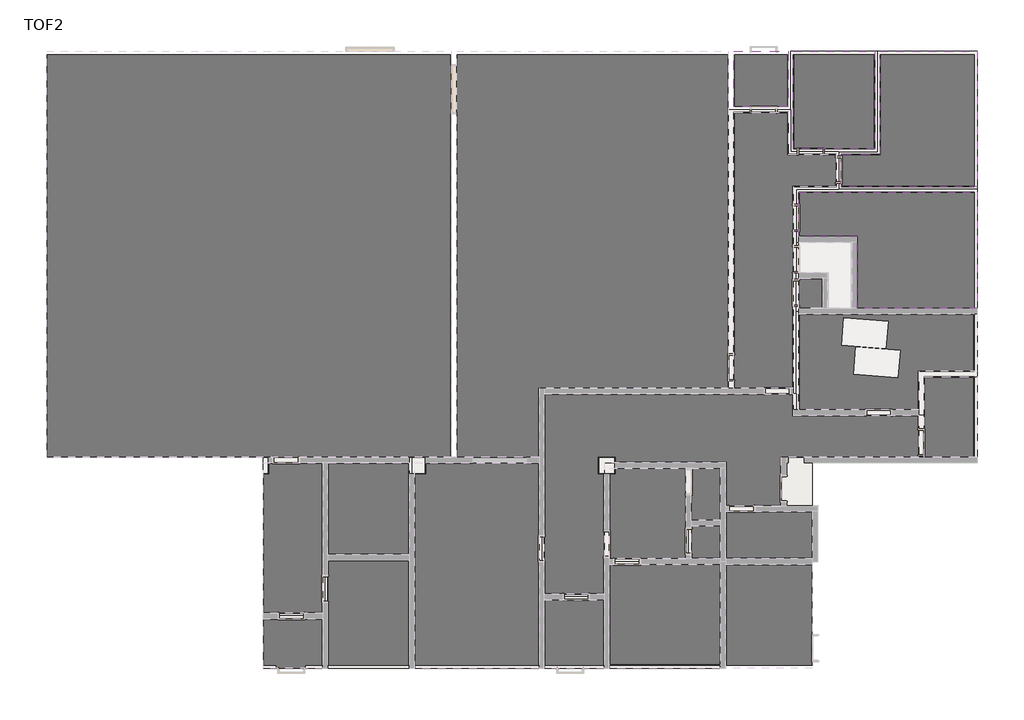
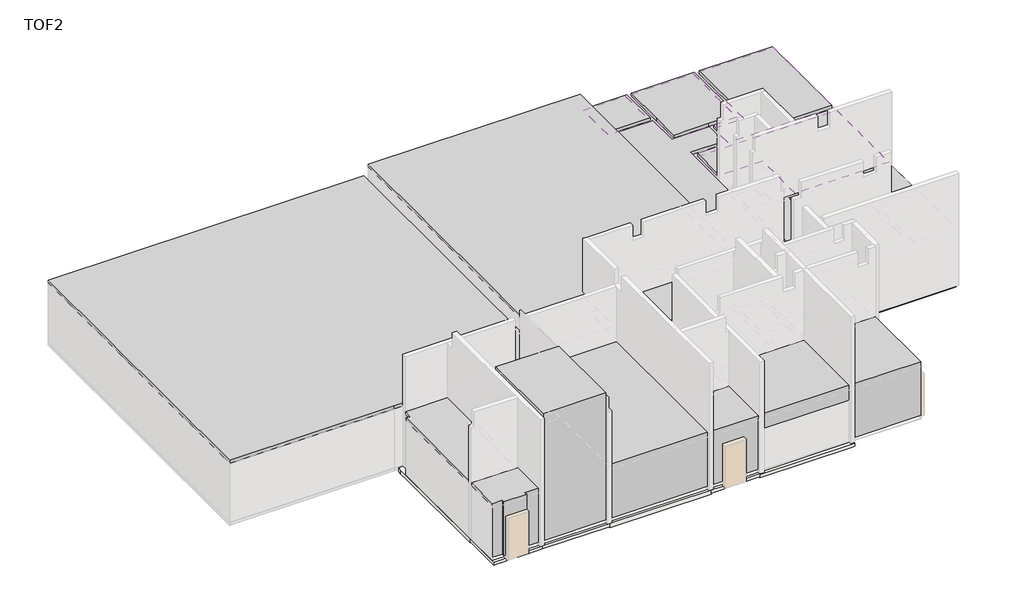
# One storey, part 5 of 5: 24 slabs, 23 proxies, 4 coverings.
"""IFC4 building model written with IfcOpenShell, lengths in millimetres."""

from ifc_helpers import new_model, si_unit, frame, origin, place, context, project, spatial, polyline, outline, extrude, faceted_brep, element, save

model = new_model("IFC4")

# Units and contexts
model_context = context("Model", 3, world=origin())
ifc_project = project(units=[si_unit("LENGTHUNIT", "METRE", prefix="MILLI")], contexts=[model_context])

# Site, building, storey
site = spatial("IfcSite", under=ifc_project)
building = spatial("IfcBuilding", under=site)
storey = spatial("IfcBuildingStorey", under=building, Name="TOF2", Elevation=999.9618634)

# Proxies
placement = place(None, origin())
element("IfcBuildingElementProxy", 1, Name="Generic Models", at=placement, inside=storey, context=model_context, shape_type="SweptSolid", body=[
    extrude(outline(polyline([(18312.0, 23473.5208589), (33238.0, 23473.5208589), (33238.0, 8611.5208589), (26100.0, 8611.5208589), (18312.0, 8611.5208589), (18312.0, 23473.5208589)])), frame((0.0, 0.0, 1149.9618634), z_axis=(0.0, 0.0, 1.0), x_axis=(1.0, 0.0, 0.0)), (0.0, 0.0, 1.0), 3000.0),
])
element("IfcBuildingElementProxy", 2, Name="Generic Models", at=placement, inside=storey, context=model_context, shape_type="SweptSolid", body=[
    extrude(outline(polyline([(36488.0, 925.5208589), (31912.0, 925.5208589), (31912.0, 4899.0208589), (31912.0, 7987.5208589), (32312.0, 7987.5208589), (32312.0, 8387.5208589), (33350.0, 8387.5208589), (36488.0, 8387.5208589), (36488.0, 3443.8249516), (36488.0, 925.5208589)])), frame((0.0, 0.0, 1156.9618634), z_axis=(0.0, 0.0, 1.0), x_axis=(1.0, 0.0, 0.0)), (0.0, 0.0, 1.0), 2693.0),
])
element("IfcBuildingElementProxy", 3, Name="Generic Models", at=placement, inside=storey, context=model_context, shape_type="SweptSolid", body=[
    extrude(outline(polyline([(33462.0, 23473.5208589), (43488.0, 23473.5208589), (43488.0, 11161.5208589), (36488.0, 11161.5208589), (36488.0, 8611.5208589), (33462.0, 8611.5208589), (33462.0, 23473.5208589)])), frame((0.0, 0.0, 1149.9618634), z_axis=(0.0, 0.0, 1.0), x_axis=(1.0, 0.0, 0.0)), (0.0, 0.0, 1.0), 3500.0),
])
element("IfcBuildingElementProxy", 4, Name="Generic Models", at=placement, inside=storey, context=model_context, shape_type="SweptSolid", body=[
    extrude(outline(polyline([(39107.0, 932.5208589), (39107.0, 3443.8249516), (39107.0, 4642.5208589), (43193.0, 4642.5208589), (43193.0, 932.5208589), (39107.0, 932.5208589)])), frame((0.0, 0.0, 1199.9618634), z_axis=(0.0, 0.0, 1.0), x_axis=(1.0, 0.0, 0.0)), (0.0, 0.0, 1.0), 2650.0),
])
element("IfcBuildingElementProxy", 5, Name="Generic Models", at=placement, inside=storey, context=model_context, shape_type="SweptSolid", body=[
    extrude(outline(polyline([(39307.0, 7992.5208589), (39307.0, 8197.5208589), (41918.0, 8197.5208589), (41918.0, 6174.5208589), (41918.0, 4856.5208589), (39107.0, 4856.5208589), (39107.0, 7992.5208589), (39307.0, 7992.5208589)])), frame((0.0, 0.0, 1149.9618634), z_axis=(0.0, 0.0, 1.0), x_axis=(1.0, 0.0, 0.0)), (0.0, 0.0, 1.0), 2700.0),
])
element("IfcBuildingElementProxy", 6, Name="Generic Models", at=placement, inside=storey, context=model_context, shape_type="SweptSolid", body=[
    extrude(outline(polyline([(42132.0, 8197.5208589), (43193.0, 8197.5208589), (43193.0, 6699.5208589), (43193.0, 6281.5208589), (42132.0, 6281.5208589), (42132.0, 8197.5208589)])), frame((0.0, 0.0, 1199.9618634), z_axis=(0.0, 0.0, 1.0), x_axis=(1.0, 0.0, 0.0)), (0.0, 0.0, 1.0), 2650.0),
])
element("IfcBuildingElementProxy", 7, Name="Generic Models", at=placement, inside=storey, context=model_context, shape_type="SweptSolid", body=[
    extrude(outline(polyline([(43188.0, 4861.5208589), (42137.0, 4861.5208589), (42137.0, 6062.5208589), (43188.0, 6062.5208589), (43188.0, 4861.5208589)])), frame((0.0, 0.0, 1149.9618634), z_axis=(0.0, 0.0, 1.0), x_axis=(1.0, 0.0, 0.0)), (0.0, 0.0, 1.0), 2700.0),
])
element("IfcBuildingElementProxy", 8, Name="Generic Models", at=placement, inside=storey, context=model_context, shape_type="SweptSolid", body=[
    extrude(outline(polyline([(52567.0, 8606.5208589), (50732.0, 8606.5208589), (50732.0, 10249.5208589), (50732.0, 11567.5208589), (52567.0, 11567.5208589), (52567.0, 8606.5208589)])), frame((0.0, 0.0, 1199.9618634), z_axis=(0.0, 0.0, 1.0), x_axis=(1.0, 0.0, 0.0)), (0.0, 0.0, 1.0), 2650.0),
])
element("IfcBuildingElementProxy", 9, Name="Generic Models", at=placement, inside=storey, context=model_context, shape_type="SweptSolid", body=[
    extrude(outline(polyline([(52574.0, 23473.5208589), (52574.0, 18611.5208589), (47687.0, 18611.5208589), (47687.0, 19787.5208589), (49112.0, 19787.5208589), (49112.0, 23473.5208589), (52574.0, 23473.5208589)])), frame((0.0, 0.0, 1156.9618634), z_axis=(0.0, 0.0, 1.0), x_axis=(1.0, 0.0, 0.0)), (0.0, 0.0, 1.0), 2693.0),
])
element("IfcBuildingElementProxy", 10, Name="Generic Models", at=placement, inside=storey, context=model_context, shape_type="SweptSolid", body=[
    extrude(outline(polyline([(43712.0, 23473.5208589), (45688.0, 23473.5208589), (45688.0, 21561.5208589), (43712.0, 21561.5208589), (43712.0, 23473.5208589)])), frame((0.0, 0.0, 1156.9618634), z_axis=(0.0, 0.0, 1.0), x_axis=(1.0, 0.0, 0.0)), (0.0, 0.0, 1.0), 2693.0),
])
element("IfcBuildingElementProxy", 11, Name="Generic Models", at=placement, inside=storey, context=model_context, shape_type="SweptSolid", body=[
    extrude(outline(polyline([(45883.0, 11161.5208589), (43712.0, 11161.5208589), (43712.0, 21337.5208589), (45688.0, 21337.5208589), (45688.0, 19787.5208589), (47463.0, 19787.5208589), (47463.0, 18611.5208589), (45883.0, 18611.5208589), (45883.0, 16649.5208589), (45883.0, 15314.5208589), (45883.0, 13999.5208589), (45883.0, 11161.5208589)])), frame((0.0, 0.0, 1156.9618634), z_axis=(0.0, 0.0, 1.0), x_axis=(1.0, 0.0, 0.0)), (0.0, 0.0, 1.0), 2693.0),
])
element("IfcBuildingElementProxy", 12, Name="Generic Models", at=placement, inside=storey, context=model_context, shape_type="SweptSolid", body=[
    extrude(outline(polyline([(45912.0, 23473.5208589), (48888.0, 23473.5208589), (48888.0, 20011.5208589), (47575.0, 20011.5208589), (45912.0, 20011.5208589), (45912.0, 21449.5208589), (45912.0, 23473.5208589)])), frame((0.0, 0.0, 1156.9618634), z_axis=(0.0, 0.0, 1.0), x_axis=(1.0, 0.0, 0.0)), (0.0, 0.0, 1.0), 2693.0),
])
element("IfcBuildingElementProxy", 13, Name="Generic Models", at=placement, inside=storey, context=model_context, shape_type="SweptSolid", body=[
    extrude(outline(polyline([(50513.0, 10361.5208589), (46107.0, 10361.5208589), (46107.0, 13887.5208589), (52562.0, 13887.5208589), (52562.0, 11786.5208589), (50513.0, 11786.5208589), (50513.0, 10361.5208589)]), holes=[polyline([(47685.4846295, 12746.0331648), (49320.3101517, 12615.8582361), (49401.2726074, 13632.6399633), (47766.4470852, 13762.814892), (47685.4846295, 12746.0331648)]), polyline([(48126.4248192, 11673.6441948), (49761.2503413, 11543.4692661), (49842.212797, 12560.2509933), (48207.3872748, 12690.425922), (48126.4248192, 11673.6441948)])]), frame((0.0, 0.0, 1206.9618634), z_axis=(0.0, 0.0, 1.0), x_axis=(1.0, 0.0, 0.0)), (0.0, 0.0, 1.0), 2643.0),
])
element("IfcBuildingElementProxy", 14, Name="Generic Models", at=placement, inside=storey, context=model_context, shape_type="SweptSolid", body=[
    extrude(outline(polyline([(52574.0, 18387.5208589), (52574.0, 14111.5208589), (48262.0, 14111.5208589), (48262.0, 16761.5208589), (46107.0, 16761.5208589), (46107.0, 18387.5208589), (52574.0, 18387.5208589)])), frame((0.0, 0.0, 1156.9618634), z_axis=(0.0, 0.0, 1.0), x_axis=(1.0, 0.0, 0.0)), (0.0, 0.0, 1.0), 2693.0),
])
element("IfcBuildingElementProxy", 15, Name="Generic Models", at=placement, inside=storey, context=model_context, shape_type="SweptSolid", body=[
    extrude(outline(polyline([(46107.0, 14111.5208589), (46107.0, 15202.5208589), (46963.0, 15202.5208589), (46963.0, 14111.5208589), (46107.0, 14111.5208589)])), frame((0.0, 0.0, 1156.9618634), z_axis=(0.0, 0.0, 1.0), x_axis=(1.0, 0.0, 0.0)), (0.0, 0.0, 1.0), 2693.0),
])
element("IfcBuildingElementProxy", 16, Name="Generic Models", at=placement, inside=storey, context=model_context, shape_type="SweptSolid", body=[
    extrude(outline(polyline([(43412.0, 6587.5208589), (46588.0, 6587.5208589), (46588.0, 4861.5208589), (43412.0, 4861.5208589), (43412.0, 6587.5208589)])), frame((0.0, 0.0, 1156.9618634), z_axis=(0.0, 0.0, 1.0), x_axis=(1.0, 0.0, 0.0)), (0.0, 0.0, 1.0), 2693.0),
])
element("IfcBuildingElementProxy", 17, Name="Generic Models", at=placement, inside=storey, context=model_context, shape_type="SweptSolid", body=[
    extrude(outline(polyline([(46588.0, 925.5208589), (43412.0, 925.5208589), (43412.0, 4637.5208589), (46588.0, 4637.5208589), (46588.0, 925.5208589)])), frame((0.0, 0.0, 1156.9618634), z_axis=(0.0, 0.0, 1.0), x_axis=(1.0, 0.0, 0.0)), (0.0, 0.0, 1.0), 2693.0),
])
element("IfcBuildingElementProxy", 18, Name="Generic Models", at=placement, inside=storey, context=model_context, shape_type="SweptSolid", body=[
    extrude(outline(polyline([(31688.0, 925.5208589), (28712.0, 925.5208589), (28712.0, 4787.0208589), (31688.0, 4787.0208589), (31688.0, 925.5208589)])), frame((0.0, 0.0, 1156.9618634), z_axis=(0.0, 0.0, 1.0), x_axis=(1.0, 0.0, 0.0)), (0.0, 0.0, 1.0), 6343.0),
])
element("IfcBuildingElementProxy", 19, Name="Generic Models", at=placement, inside=storey, context=model_context, shape_type="SweptSolid", body=[
    extrude(outline(polyline([(28712.0, 8387.5208589), (31688.0, 8387.5208589), (31688.0, 7999.5208589), (31688.0, 5011.0208589), (28712.0, 5011.0208589), (28712.0, 8387.5208589)])), frame((0.0, 0.0, 1156.9618634), z_axis=(0.0, 0.0, 1.0), x_axis=(1.0, 0.0, 0.0)), (0.0, 0.0, 1.0), 2693.0),
])
element("IfcBuildingElementProxy", 20, Name="Generic Models", at=placement, inside=storey, context=model_context, shape_type="Brep", body=[
    faceted_brep([(26787.0, 925.5208589, 1156.9618634), (26850.0, 925.5208589, 1156.9618634), (26850.0, 925.5208589, 1149.9618634), (26787.0, 925.5208589, 1149.9618634), (26850.0, 799.5208589, 1156.9618634), (26312.0, 925.5208589, 1156.9618634), (26312.0, 2625.0208589, 1156.9618634), (28488.0, 2625.0208589, 1156.9618634), (28488.0, 925.5208589, 1156.9618634), (27855.0, 925.5208589, 1156.9618634), (27855.0, 799.5208589, 1156.9618634), (26787.0, 925.5208589, 3849.9618634), (26312.0, 925.5208589, 3849.9618634), (26850.0, 799.5208589, 1149.9618634), (26787.0, 799.5208589, 1149.9618634), (26787.0, 799.5208589, 3849.9618634), (27855.0, 799.5208589, 3849.9618634), (26312.0, 2625.0208589, 3849.9618634), (28488.0, 2625.0208589, 3849.9618634), (28488.0, 925.5208589, 3849.9618634), (27855.0, 925.5208589, 3849.9618634)], [[[0, 1, 2, 3]], [[4, 1, 0, 5, 6, 7, 8, 9, 10]], [[11, 12, 5, 0]], [[1, 4, 13, 2]], [[14, 3, 2, 13]], [[3, 14, 15, 11, 0]], [[15, 14, 13, 4, 10, 16]], [[12, 17, 6, 5]], [[17, 18, 7, 6]], [[18, 19, 8, 7]], [[19, 20, 9, 8]], [[20, 16, 10, 9]], [[11, 15, 16, 20, 19, 18, 17, 12]]]),
])
element("IfcBuildingElementProxy", 21, Name="Generic Models", at=placement, inside=storey, context=model_context, shape_type="SweptSolid", body=[
    extrude(outline(polyline([(26512.0, 7987.5208589), (26512.0, 8387.5208589), (28488.0, 8387.5208589), (28488.0, 4899.0208589), (28488.0, 2849.0208589), (26312.0, 2849.0208589), (26312.0, 7987.5208589), (26512.0, 7987.5208589)])), frame((0.0, 0.0, 1156.9618634), z_axis=(0.0, 0.0, 1.0), x_axis=(1.0, 0.0, 0.0)), (0.0, 0.0, 1.0), 2693.0),
])
element("IfcBuildingElementProxy", 22, Name="Generic Models", at=placement, inside=storey, context=model_context, shape_type="SweptSolid", body=[
    extrude(outline(polyline([(39312.0, 8416.5208589), (39312.0, 8611.5208589), (38688.0, 8611.5208589), (38688.0, 7987.5208589), (38888.0, 7987.5208589), (38888.0, 3555.8249516), (36712.0, 3555.8249516), (36712.0, 8499.5208589), (36712.0, 10937.5208589), (43600.0, 10937.5208589), (45883.0, 10937.5208589), (45883.0, 10137.5208589), (50513.0, 10137.5208589), (50513.0, 8611.5208589), (45428.0, 8611.5208589), (45428.0, 6811.5208589), (43412.0, 6811.5208589), (43412.0, 8416.5208589), (39312.0, 8416.5208589)])), frame((0.0, 0.0, 1156.9618634), z_axis=(0.0, 0.0, 1.0), x_axis=(1.0, 0.0, 0.0)), (0.0, 0.0, 1.0), 2693.0),
])
element("IfcBuildingElementProxy", 23, Name="Generic Models", at=placement, inside=storey, context=model_context, shape_type="SweptSolid", body=[
    extrude(outline(polyline([(38888.0, 925.5208589), (36712.0, 925.5208589), (36712.0, 3331.8249516), (38888.0, 3331.8249516), (38888.0, 925.5208589)])), frame((0.0, 0.0, 1156.9618634), z_axis=(0.0, 0.0, 1.0), x_axis=(1.0, 0.0, 0.0)), (0.0, 0.0, 1.0), 2693.0),
])

# Coverings
element("IfcCovering", 24, ObjectType="H_CE_AR_B09_Acoustic Ceiling_T Bar_600x600x9T", at=placement, inside=storey, context=model_context, shape_type="SweptSolid", body=[
    extrude(outline(polyline([(43700.0, 23599.5208589), (45700.0, 23599.5208589), (45700.0, 21549.5208589), (43700.0, 21549.5208589), (43700.0, 23599.5208589)])), frame((0.0, 0.0, 3699.9618634), z_axis=(0.0, 0.0, 1.0), x_axis=(1.0, 0.0, 0.0)), (0.0, 0.0, 1.0), 9.0),
])
element("IfcCovering", 25, ObjectType="H_CE_AR_B09_Acoustic Ceiling_T Bar_600x600x9T", at=placement, inside=storey, context=model_context, shape_type="SweptSolid", body=[
    extrude(outline(polyline([(45900.0, 23599.5208589), (48900.0, 23599.5208589), (48900.0, 19999.5208589), (45900.0, 19999.5208589), (45900.0, 23599.5208589)])), frame((0.0, 0.0, 3699.9618634), z_axis=(0.0, 0.0, 1.0), x_axis=(1.0, 0.0, 0.0)), (0.0, 0.0, 1.0), 9.0),
])
element("IfcCovering", 26, ObjectType="H_CE_AR_B09_Acoustic Ceiling_T Bar_600x600x9T", at=placement, inside=storey, context=model_context, shape_type="SweptSolid", body=[
    extrude(outline(polyline([(49100.0, 23599.5208589), (52700.0, 23599.5208589), (52700.0, 18599.5208589), (47675.0, 18599.5208589), (47675.0, 19799.5208589), (49100.0, 19799.5208589), (49100.0, 23599.5208589)])), frame((0.0, 0.0, 3699.9618634), z_axis=(0.0, 0.0, 1.0), x_axis=(1.0, 0.0, 0.0)), (0.0, 0.0, 1.0), 9.0),
])
element("IfcCovering", 27, ObjectType="H_CE_AR_B09_Acoustic Ceiling_T Bar_600x600x9T", at=placement, inside=storey, context=model_context, shape_type="SweptSolid", body=[
    extrude(outline(polyline([(52700.0, 18399.5208589), (52700.0, 14099.5208589), (48250.0, 14099.5208589), (48250.0, 16749.5208589), (46095.0, 16749.5208589), (46095.0, 18399.5208589), (52700.0, 18399.5208589)])), frame((0.0, 0.0, 3699.9618634), z_axis=(0.0, 0.0, 1.0), x_axis=(1.0, 0.0, 0.0)), (0.0, 0.0, 1.0), 9.0),
])

# Slabs
element("IfcSlab", 28, ObjectType="H_SF_AR_S17_SOG T200_GS1", at=placement, inside=storey, context=model_context, shape_type="Brep", body=[
    faceted_brep([(33350.0, 8599.5208589, 799.9618634), (36600.0, 8599.5208589, 799.9618634), (36600.0, 3443.8249516, 799.9618634), (36600.0, 925.5208589, 799.9618634), (36600.0, 799.5208589, 799.9618634), (31800.0, 799.5208589, 799.9618634), (31800.0, 925.5208589, 799.9618634), (31800.0, 4899.0208589, 799.9618634), (31800.0, 8599.5208589, 799.9618634), (32300.0, 8599.5208589, 799.9618634), (33350.0, 8599.5208589, 999.9618634), (31800.0, 8599.5208589, 999.9618634), (31800.0, 4899.0208589, 999.9618634), (31800.0, 799.5208589, 999.9618634), (31900.0, 799.5208589, 999.9618634), (36500.0, 799.5208589, 999.9618634), (36600.0, 799.5208589, 999.9618634), (36600.0, 3443.8249516, 999.9618634), (36600.0, 8599.5208589, 999.9618634), (36500.0, 8599.5208589, 999.9618634), (36600.0, 799.5208589, 849.9618634), (31800.0, 799.5208589, 849.9618634)], [[[0, 1, 2, 3, 4, 5, 6, 7, 8, 9]], [[10, 11, 12, 13, 14, 15, 16, 17, 18, 19]], [[1, 0, 10, 19, 18]], [[2, 1, 18, 17]], [[4, 3, 2, 17, 16, 20]], [[5, 4, 20, 16, 15, 14, 13, 21]], [[7, 6, 5, 21, 13, 12]], [[8, 7, 12, 11]], [[0, 9, 8, 11, 10]]]),
])
element("IfcSlab", 29, ObjectType="H_SF_AR_S17_SOG T150_GS1", at=placement, inside=storey, context=model_context, shape_type="Brep", body=[
    faceted_brep([(38900.0, 799.5208589, 799.9618634), (38900.0, 925.5208589, 799.9618634), (38900.0, 3443.8249516, 799.9618634), (38900.0, 4749.5208589, 799.9618634), (42025.0, 4749.5208589, 799.9618634), (43400.0, 4749.5208589, 799.9618634), (43400.0, 4649.5208589, 799.9618634), (43400.0, 925.5208589, 799.9618634), (43400.0, 799.5208589, 799.9618634), (43200.0, 799.5208589, 799.9618634), (38900.0, 799.5208589, 949.9618634), (43200.0, 799.5208589, 949.9618634), (43400.0, 799.5208589, 949.9618634), (43400.0, 925.5208589, 949.9618634), (43400.0, 4749.5208589, 949.9618634), (42025.0, 4749.5208589, 949.9618634), (38900.0, 4749.5208589, 949.9618634), (38900.0, 3443.8249516, 949.9618634), (38900.0, 925.5208589, 949.9618634), (38900.0, 799.5208589, 849.9618634)], [[[0, 1, 2, 3, 4, 5, 6, 7, 8, 9]], [[10, 11, 12, 13, 14, 15, 16, 17, 18]], [[2, 1, 0, 19, 10, 18, 17]], [[3, 2, 17, 16]], [[4, 3, 16, 15]], [[5, 4, 15, 14]], [[8, 7, 6, 5, 14, 13, 12]], [[0, 9, 8, 12, 11, 10, 19]]]),
])
element("IfcSlab", 30, ObjectType="H_SF_AR_S17_SOG T150_GS1", at=placement, inside=storey, context=model_context, shape_type="SweptSolid", body=[
    extrude(outline(polyline([(38900.0, 4749.5208589), (38900.0, 8404.5208589), (42025.0, 8404.5208589), (42025.0, 6174.5208589), (42025.0, 4749.5208589), (38900.0, 4749.5208589)])), frame((0.0, 0.0, 799.9618634), z_axis=(0.0, 0.0, 1.0), x_axis=(1.0, 0.0, 0.0)), (0.0, 0.0, 1.0), 150.0),
])
element("IfcSlab", 31, ObjectType="H_SF_AR_S17_SOG T200_GS1", at=placement, inside=storey, context=model_context, shape_type="Brep", body=[
    faceted_brep([(42025.0, 8404.5208589, 799.9618634), (43400.0, 8404.5208589, 799.9618634), (43400.0, 6699.5208589, 799.9618634), (43400.0, 6174.5208589, 799.9618634), (42025.0, 6174.5208589, 799.9618634), (42025.0, 8404.5208589, 999.9618634), (42025.0, 6174.5208589, 999.9618634), (43400.0, 6174.5208589, 999.9618634), (43400.0, 6699.5208589, 999.9618634), (43400.0, 8404.5208589, 999.9618634), (42025.0, 8404.5208589, 949.9618634), (43400.0, 6174.5208589, 949.9618634), (42025.0, 6174.5208589, 949.9618634)], [[[0, 1, 2, 3, 4]], [[5, 6, 7, 8, 9]], [[1, 0, 10, 5, 9]], [[2, 1, 9, 8]], [[3, 2, 8, 7, 11]], [[4, 3, 11, 7, 6, 12]], [[0, 4, 12, 6, 5, 10]]]),
])
element("IfcSlab", 32, ObjectType="H_SF_AR_S17_SOG T150_GS1", at=placement, inside=storey, context=model_context, shape_type="Brep", body=[
    faceted_brep([(43400.0, 4749.5208589, 799.9618634), (42025.0, 4749.5208589, 799.9618634), (42025.0, 6174.5208589, 799.9618634), (43400.0, 6174.5208589, 799.9618634), (43400.0, 4849.5208589, 799.9618634), (43400.0, 4749.5208589, 949.9618634), (43400.0, 4849.5208589, 949.9618634), (43400.0, 6174.5208589, 949.9618634), (42025.0, 6174.5208589, 949.9618634), (42025.0, 4749.5208589, 949.9618634)], [[[0, 1, 2, 3, 4]], [[5, 6, 7, 8, 9]], [[1, 0, 5, 9]], [[2, 1, 9, 8]], [[3, 2, 8, 7]], [[0, 4, 3, 7, 6, 5]]]),
])
element("IfcSlab", 33, ObjectType="H_SF_AR_S17_SOG T150_GS1", at=placement, inside=storey, context=model_context, shape_type="Brep", body=[
    faceted_brep([(52700.0, 8599.5208589, 799.9618634), (52574.0, 8599.5208589, 799.9618634), (50725.0, 8599.5208589, 799.9618634), (50725.0, 10149.5208589, 799.9618634), (50725.0, 10249.5208589, 799.9618634), (50725.0, 11574.5208589, 799.9618634), (52574.0, 11574.5208589, 799.9618634), (52700.0, 11574.5208589, 799.9618634), (52700.0, 8599.5208589, 949.9618634), (52700.0, 11574.5208589, 949.9618634), (52574.0, 11574.5208589, 949.9618634), (50725.0, 11574.5208589, 949.9618634), (50725.0, 10249.5208589, 949.9618634), (50725.0, 8599.5208589, 949.9618634), (52574.0, 8599.5208589, 949.9618634), (50725.0, 11574.5208589, 849.9618634), (52700.0, 11574.5208589, 849.9618634)], [[[0, 1, 2, 3, 4, 5, 6, 7]], [[8, 9, 10, 11, 12, 13, 14]], [[2, 1, 0, 8, 14, 13]], [[4, 3, 2, 13, 12]], [[5, 4, 12, 11, 15]], [[7, 6, 5, 15, 11, 10, 9, 16]], [[0, 7, 16, 9, 8]]]),
])
element("IfcSlab", 34, ObjectType="H_SF_AR_S17_SOG T150_GS1", at=placement, inside=storey, context=model_context, shape_type="Brep", body=[
    faceted_brep([(52700.0, 18499.5208589, 849.9618634), (47575.0, 18499.5208589, 849.9618634), (47575.0, 19899.5208589, 849.9618634), (49000.0, 19899.5208589, 849.9618634), (49000.0, 23599.5208589, 849.9618634), (49100.0, 23599.5208589, 849.9618634), (52574.0, 23599.5208589, 849.9618634), (52700.0, 23599.5208589, 849.9618634), (52700.0, 18599.5208589, 849.9618634), (52700.0, 18499.5208589, 999.9618634), (52700.0, 18599.5208589, 999.9618634), (52700.0, 23599.5208589, 999.9618634), (52574.0, 23599.5208589, 999.9618634), (49100.0, 23599.5208589, 999.9618634), (49000.0, 23599.5208589, 999.9618634), (49000.0, 19899.5208589, 999.9618634), (47575.0, 19899.5208589, 999.9618634), (47575.0, 18499.5208589, 999.9618634)], [[[0, 1, 2, 3, 4, 5, 6, 7, 8]], [[9, 10, 11, 12, 13, 14, 15, 16, 17]], [[1, 0, 9, 17]], [[2, 1, 17, 16]], [[3, 2, 16, 15]], [[4, 3, 15, 14]], [[7, 6, 5, 4, 14, 13, 12, 11]], [[0, 8, 7, 11, 10, 9]]]),
])
element("IfcSlab", 35, ObjectType="H_SF_AR_S17_SOG T150_GS1", at=placement, inside=storey, context=model_context, shape_type="Brep", body=[
    faceted_brep([(46000.0, 10949.5208589, 849.9618634), (43500.0, 10949.5208589, 849.9618634), (43500.0, 11149.5208589, 849.9618634), (43500.0, 21449.5208589, 849.9618634), (43700.0, 21449.5208589, 849.9618634), (45800.0, 21449.5208589, 849.9618634), (45800.0, 19899.5208589, 849.9618634), (47575.0, 19899.5208589, 849.9618634), (47575.0, 18499.5208589, 849.9618634), (46000.0, 18499.5208589, 849.9618634), (46000.0, 16649.5208589, 849.9618634), (46000.0, 16549.5208589, 849.9618634), (46000.0, 15414.5208589, 849.9618634), (46000.0, 15412.0208589, 849.9618634), (46000.0, 15314.5208589, 849.9618634), (46000.0, 13999.5208589, 849.9618634), (46000.0, 11149.5208589, 849.9618634), (46000.0, 10949.5208589, 999.9618634), (46000.0, 13999.5208589, 999.9618634), (46000.0, 15314.5208589, 999.9618634), (46000.0, 15412.0208589, 999.9618634), (46000.0, 16412.0208589, 999.9618634), (46000.0, 16549.5208589, 999.9618634), (46000.0, 16649.5208589, 999.9618634), (46000.0, 18499.5208589, 999.9618634), (47575.0, 18499.5208589, 999.9618634), (47575.0, 19899.5208589, 999.9618634), (45800.0, 19899.5208589, 999.9618634), (45800.0, 21449.5208589, 999.9618634), (43700.0, 21449.5208589, 999.9618634), (43500.0, 21449.5208589, 999.9618634), (43500.0, 12424.5208589, 999.9618634), (43500.0, 11424.5208589, 999.9618634), (43500.0, 11149.5208589, 999.9618634), (43500.0, 10949.5208589, 999.9618634), (44800.0, 10949.5208589, 999.9618634), (45800.0, 10949.5208589, 999.9618634), (45895.0, 10949.5208589, 999.9618634)], [[[0, 1, 2, 3, 4, 5, 6, 7, 8, 9, 10, 11, 12, 13, 14, 15, 16]], [[17, 18, 19, 20, 21, 22, 23, 24, 25, 26, 27, 28, 29, 30, 31, 32, 33, 34, 35, 36, 37]], [[1, 0, 17, 37, 36, 35, 34]], [[3, 2, 1, 34, 33, 32, 31, 30]], [[5, 4, 3, 30, 29, 28]], [[6, 5, 28, 27]], [[7, 6, 27, 26]], [[8, 7, 26, 25]], [[9, 8, 25, 24]], [[10, 9, 24, 23]], [[14, 13, 12, 11, 10, 23, 22, 21, 20, 19]], [[15, 14, 19, 18]], [[0, 16, 15, 18, 17]]]),
])
element("IfcSlab", 36, ObjectType="H_SF_AR_S17_SOG T150_GS1", at=placement, inside=storey, context=model_context, shape_type="Brep", body=[
    faceted_brep([(47575.0, 19899.5208589, 849.9618634), (45800.0, 19899.5208589, 849.9618634), (45800.0, 21449.5208589, 849.9618634), (45800.0, 23599.5208589, 849.9618634), (45900.0, 23599.5208589, 849.9618634), (48900.0, 23599.5208589, 849.9618634), (49000.0, 23599.5208589, 849.9618634), (49000.0, 19899.5208589, 849.9618634), (45800.0, 19899.5208589, 999.9618634), (47575.0, 19899.5208589, 999.9618634), (49000.0, 19899.5208589, 999.9618634), (49000.0, 23599.5208589, 999.9618634), (48900.0, 23599.5208589, 999.9618634), (45900.0, 23599.5208589, 999.9618634), (45800.0, 23599.5208589, 999.9618634), (45800.0, 21449.5208589, 999.9618634)], [[[0, 1, 2, 3, 4, 5, 6, 7]], [[8, 9, 10, 11, 12, 13, 14, 15]], [[1, 0, 9, 8]], [[2, 1, 8, 15]], [[3, 2, 15, 14]], [[6, 5, 4, 3, 14, 13, 12, 11]], [[7, 6, 11, 10]], [[0, 7, 10, 9]]]),
])
element("IfcSlab", 37, ObjectType="H_SF_AR_S17_SOG T150_GS1", at=placement, inside=storey, context=model_context, shape_type="Brep", body=[
    faceted_brep([(50725.0, 10149.5208589, 849.9618634), (50525.0, 10149.5208589, 849.9618634), (46000.0, 10149.5208589, 849.9618634), (46000.0, 10349.5208589, 849.9618634), (46000.0, 10949.5208589, 849.9618634), (46000.0, 11049.5208589, 849.9618634), (46000.0, 11149.5208589, 849.9618634), (46000.0, 13999.5208589, 849.9618634), (47075.0, 13999.5208589, 849.9618634), (47175.0, 13999.5208589, 849.9618634), (48050.0, 13999.5208589, 849.9618634), (48150.0, 13999.5208589, 849.9618634), (52700.0, 13999.5208589, 849.9618634), (52700.0, 11774.5208589, 849.9618634), (52700.0, 11574.5208589, 849.9618634), (50725.0, 11574.5208589, 849.9618634), (50725.0, 10249.5208589, 849.9618634), (46000.0, 10149.5208589, 999.9618634), (50725.0, 10149.5208589, 999.9618634), (50725.0, 11574.5208589, 999.9618634), (52700.0, 11574.5208589, 999.9618634), (52700.0, 11774.5208589, 999.9618634), (52700.0, 13899.5208589, 999.9618634), (52700.0, 13999.5208589, 999.9618634), (48150.0, 13999.5208589, 999.9618634), (48050.0, 13999.5208589, 999.9618634), (47175.0, 13999.5208589, 999.9618634), (47075.0, 13999.5208589, 999.9618634), (46000.0, 13999.5208589, 999.9618634), (46000.0, 11049.5208589, 999.9618634), (46000.0, 10949.5208589, 999.9618634), (50725.0, 10149.5208589, 949.9618634), (52700.0, 11574.5208589, 949.9618634), (50725.0, 11574.5208589, 949.9618634)], [[[0, 1, 2, 3, 4, 5, 6, 7, 8, 9, 10, 11, 12, 13, 14, 15, 16]], [[17, 18, 19, 20, 21, 22, 23, 24, 25, 26, 27, 28, 29, 30]], [[2, 1, 0, 31, 18, 17]], [[2, 17, 30, 29, 5, 4, 3]], [[7, 6, 5, 29, 28]], [[8, 7, 28, 27]], [[11, 10, 9, 8, 27, 26, 25, 24]], [[12, 11, 24, 23]], [[14, 13, 12, 23, 22, 21, 20, 32]], [[15, 14, 32, 20, 19, 33]], [[19, 18, 31, 0, 16, 15, 33]]]),
])
element("IfcSlab", 38, ObjectType="H_SF_AR_S17_SOG T150_GS1", at=placement, inside=storey, context=model_context, shape_type="Brep", body=[
    faceted_brep([(46000.0, 18499.5208589, 849.9618634), (47575.0, 18499.5208589, 849.9618634), (52700.0, 18499.5208589, 849.9618634), (52700.0, 18399.5208589, 849.9618634), (52700.0, 13999.5208589, 849.9618634), (48050.0, 13999.5208589, 849.9618634), (48050.0, 16549.5208589, 849.9618634), (46095.0, 16549.5208589, 849.9618634), (46000.0, 16549.5208589, 849.9618634), (46000.0, 16649.5208589, 849.9618634), (47575.0, 18499.5208589, 999.9618634), (46000.0, 18499.5208589, 999.9618634), (46000.0, 16649.5208589, 999.9618634), (46000.0, 16549.5208589, 999.9618634), (46095.0, 16549.5208589, 999.9618634), (48050.0, 16549.5208589, 999.9618634), (48050.0, 13999.5208589, 999.9618634), (52700.0, 13999.5208589, 999.9618634), (52700.0, 14099.5208589, 999.9618634), (52700.0, 18399.5208589, 999.9618634), (52700.0, 18499.5208589, 999.9618634), (46000.0, 16549.5208589, 949.9618634), (48050.0, 13999.5208589, 949.9618634), (48050.0, 16549.5208589, 949.9618634)], [[[0, 1, 2, 3, 4, 5, 6, 7, 8, 9]], [[10, 11, 12, 13, 14, 15, 16, 17, 18, 19, 20]], [[11, 0, 9, 8, 21, 13, 12]], [[1, 0, 11, 10]], [[2, 1, 10, 20]], [[4, 3, 2, 20, 19, 18, 17]], [[5, 4, 17, 16, 22]], [[6, 5, 22, 16, 15, 23]], [[8, 7, 6, 23, 15, 14, 13, 21]]]),
])
element("IfcSlab", 39, ObjectType="H_SF_AR_S17_SOG T150_GS1", at=placement, inside=storey, context=model_context, shape_type="Brep", body=[
    faceted_brep([(46000.0, 15414.5208589, 799.9618634), (46000.0, 16549.5208589, 799.9618634), (46095.0, 16549.5208589, 799.9618634), (48050.0, 16549.5208589, 799.9618634), (48050.0, 13999.5208589, 799.9618634), (47175.0, 13999.5208589, 799.9618634), (47175.0, 15414.5208589, 799.9618634), (46095.0, 15414.5208589, 799.9618634), (46000.0, 16549.5208589, 949.9618634), (46000.0, 15414.5208589, 949.9618634), (46095.0, 15414.5208589, 949.9618634), (47175.0, 15414.5208589, 949.9618634), (47175.0, 13999.5208589, 949.9618634), (48050.0, 13999.5208589, 949.9618634), (48050.0, 16549.5208589, 949.9618634), (46095.0, 16549.5208589, 949.9618634), (46000.0, 15414.5208589, 849.9618634), (46000.0, 16549.5208589, 849.9618634), (48050.0, 16549.5208589, 849.9618634), (48050.0, 13999.5208589, 849.9618634), (47175.0, 13999.5208589, 849.9618634)], [[[0, 1, 2, 3, 4, 5, 6, 7]], [[8, 9, 10, 11, 12, 13, 14, 15]], [[1, 0, 16, 9, 8, 17]], [[3, 2, 1, 17, 8, 15, 14, 18]], [[4, 3, 18, 14, 13, 19]], [[5, 4, 19, 13, 12, 20]], [[6, 5, 20, 12, 11]], [[0, 7, 6, 11, 10, 9, 16]]]),
])
element("IfcSlab", 40, ObjectType="H_SF_AR_S17_SOG T150_GS1", at=placement, inside=storey, context=model_context, shape_type="Brep", body=[
    faceted_brep([(46000.0, 15412.0208589, 849.9618634), (46095.0, 15412.0208589, 849.9618634), (47175.0, 15412.0208589, 849.9618634), (47175.0, 13999.5208589, 849.9618634), (46000.0, 13999.5208589, 849.9618634), (46000.0, 15314.5208589, 849.9618634), (47175.0, 15412.0208589, 999.9618634), (46095.0, 15412.0208589, 999.9618634), (46000.0, 15412.0208589, 999.9618634), (46000.0, 15314.5208589, 999.9618634), (46000.0, 13999.5208589, 999.9618634), (47175.0, 13999.5208589, 999.9618634), (47175.0, 15214.5208589, 999.9618634), (47175.0, 15412.0208589, 949.9618634), (47175.0, 13999.5208589, 949.9618634)], [[[0, 1, 2, 3, 4, 5]], [[6, 7, 8, 9, 10, 11, 12]], [[8, 0, 5, 4, 10, 9]], [[2, 1, 0, 8, 7, 6, 13]], [[3, 2, 13, 6, 12, 11, 14]], [[4, 3, 14, 11, 10]]]),
])
element("IfcSlab", 41, ObjectType="H_SF_AR_S17_SOG T150_GS1", at=placement, inside=storey, context=model_context, shape_type="Brep", body=[
    faceted_brep([(31800.0, 4899.0208589, 849.9618634), (31800.0, 925.5208589, 849.9618634), (31800.0, 799.5208589, 849.9618634), (28600.0, 799.5208589, 849.9618634), (28600.0, 2737.0208589, 849.9618634), (28600.0, 4899.0208589, 849.9618634), (31800.0, 4899.0208589, 999.9618634), (28600.0, 4899.0208589, 999.9618634), (28600.0, 2737.0208589, 999.9618634), (28600.0, 799.5208589, 999.9618634), (28700.0, 799.5208589, 999.9618634), (31700.0, 799.5208589, 999.9618634), (31800.0, 799.5208589, 999.9618634)], [[[0, 1, 2, 3, 4, 5]], [[6, 7, 8, 9, 10, 11, 12]], [[2, 1, 0, 6, 12]], [[3, 2, 12, 11, 10, 9]], [[4, 3, 9, 8]], [[5, 4, 8, 7]], [[0, 5, 7, 6]]]),
])
element("IfcSlab", 42, ObjectType="H_SF_AR_S17_SOG T200_GS1", at=placement, inside=storey, context=model_context, shape_type="Brep", body=[
    faceted_brep([(28600.0, 8599.5208589, 799.9618634), (31700.0, 8599.5208589, 799.9618634), (31800.0, 8599.5208589, 799.9618634), (31800.0, 4899.0208589, 799.9618634), (28600.0, 4899.0208589, 799.9618634), (28600.0, 8599.5208589, 999.9618634), (28600.0, 4899.0208589, 999.9618634), (31800.0, 4899.0208589, 999.9618634), (31800.0, 8599.5208589, 999.9618634), (31800.0, 4899.0208589, 849.9618634), (28600.0, 4899.0208589, 849.9618634)], [[[0, 1, 2, 3, 4]], [[5, 6, 7, 8]], [[2, 1, 0, 5, 8]], [[3, 2, 8, 7, 9]], [[4, 3, 9, 7, 6, 10]], [[0, 4, 10, 6, 5]]]),
])
element("IfcSlab", 43, ObjectType="H_SF_AR_S17_SOG T150_GS1", at=placement, inside=storey, context=model_context, shape_type="Brep", body=[
    faceted_brep([(26300.0, 799.5208589, 849.9618634), (26300.0, 925.5208589, 849.9618634), (26300.0, 2737.0208589, 849.9618634), (26500.0, 2737.0208589, 849.9618634), (28600.0, 2737.0208589, 849.9618634), (28600.0, 799.5208589, 849.9618634), (27855.0, 799.5208589, 849.9618634), (26850.0, 799.5208589, 849.9618634), (26724.0, 799.5208589, 849.9618634), (26500.0, 799.5208589, 849.9618634), (26300.0, 799.5208589, 999.9618634), (26724.0, 799.5208589, 999.9618634), (26850.0, 799.5208589, 999.9618634), (27850.0, 799.5208589, 999.9618634), (27855.0, 799.5208589, 999.9618634), (28500.0, 799.5208589, 999.9618634), (28600.0, 799.5208589, 999.9618634), (28600.0, 2737.0208589, 999.9618634), (26300.0, 2737.0208589, 999.9618634), (26300.0, 925.5208589, 999.9618634)], [[[0, 1, 2, 3, 4, 5, 6, 7, 8, 9]], [[10, 11, 12, 13, 14, 15, 16, 17, 18, 19]], [[2, 1, 0, 10, 19, 18]], [[4, 3, 2, 18, 17]], [[5, 4, 17, 16]], [[0, 9, 8, 7, 6, 5, 16, 15, 14, 13, 12, 11, 10]]]),
])
element("IfcSlab", 44, ObjectType="H_SF_AR_S17_SOG T200_GS1", at=placement, inside=storey, context=model_context, shape_type="Brep", body=[
    faceted_brep([(26300.0, 8599.5208589, 799.9618634), (26500.0, 8599.5208589, 799.9618634), (28600.0, 8599.5208589, 799.9618634), (28600.0, 4899.0208589, 799.9618634), (28600.0, 2737.0208589, 799.9618634), (26500.0, 2737.0208589, 799.9618634), (26300.0, 2737.0208589, 799.9618634), (26300.0, 7999.5208589, 799.9618634), (26300.0, 8397.9255867, 799.9618634), (26300.0, 8599.5208589, 999.9618634), (26300.0, 8397.9255867, 999.9618634), (26300.0, 2737.0208589, 999.9618634), (28600.0, 2737.0208589, 999.9618634), (28600.0, 4899.0208589, 999.9618634), (28600.0, 8599.5208589, 999.9618634), (27650.0, 8599.5208589, 999.9618634), (26650.0, 8599.5208589, 999.9618634), (28600.0, 2737.0208589, 849.9618634), (26300.0, 2737.0208589, 849.9618634)], [[[0, 1, 2, 3, 4, 5, 6, 7, 8]], [[9, 10, 11, 12, 13, 14, 15, 16]], [[2, 1, 0, 9, 16, 15, 14]], [[3, 2, 14, 13]], [[4, 3, 13, 12, 17]], [[6, 5, 4, 17, 12, 11, 18]], [[8, 7, 6, 18, 11, 10]], [[0, 8, 10, 9]]]),
])
element("IfcSlab", 45, ObjectType="H_SF_AR_S17_SOG T200_GS1", at=placement, inside=storey, context=model_context, shape_type="Brep", body=[
    faceted_brep([(36600.0, 8499.5208589, 799.9618634), (36600.0, 8599.5208589, 799.9618634), (36600.0, 10799.5208589, 799.9618634), (36600.0, 11149.5208589, 799.9618634), (43500.0, 11149.5208589, 799.9618634), (43600.0, 11149.5208589, 799.9618634), (43700.0, 11149.5208589, 799.9618634), (45895.0, 11149.5208589, 799.9618634), (46000.0, 11149.5208589, 799.9618634), (46000.0, 10349.5208589, 799.9618634), (46000.0, 10149.5208589, 799.9618634), (50525.0, 10149.5208589, 799.9618634), (50725.0, 10149.5208589, 799.9618634), (50725.0, 8599.5208589, 799.9618634), (50525.0, 8599.5208589, 799.9618634), (46600.0, 8599.5208589, 799.9618634), (46600.0, 8399.5208589, 799.9618634), (46600.0, 8387.5208589, 799.9618634), (46600.0, 4849.5208589, 799.9618634), (46600.0, 4649.5208589, 799.9618634), (43400.0, 4649.5208589, 799.9618634), (43400.0, 4749.5208589, 799.9618634), (43400.0, 4849.5208589, 799.9618634), (43400.0, 6174.5208589, 799.9618634), (43400.0, 6699.5208589, 799.9618634), (43400.0, 8404.5208589, 799.9618634), (42025.0, 8404.5208589, 799.9618634), (38900.0, 8404.5208589, 799.9618634), (38900.0, 4749.5208589, 799.9618634), (38900.0, 3443.8249516, 799.9618634), (36600.0, 3443.8249516, 799.9618634), (36600.0, 11149.5208589, 999.9618634), (36600.0, 10799.5208589, 999.9618634), (36600.0, 8599.5208589, 999.9618634), (36600.0, 8499.5208589, 999.9618634), (36600.0, 3443.8249516, 999.9618634), (38900.0, 3443.8249516, 999.9618634), (38900.0, 4749.5208589, 999.9618634), (38900.0, 8404.5208589, 999.9618634), (42025.0, 8404.5208589, 999.9618634), (43400.0, 8404.5208589, 999.9618634), (43400.0, 6699.5208589, 999.9618634), (43400.0, 6174.5208589, 999.9618634), (43400.0, 4849.5208589, 999.9618634), (43400.0, 4649.5208589, 999.9618634), (46600.0, 4649.5208589, 999.9618634), (46600.0, 4749.5208589, 999.9618634), (46600.0, 4849.5208589, 999.9618634), (46600.0, 8387.5208589, 999.9618634), (46600.0, 8399.5208589, 999.9618634), (46600.0, 8599.5208589, 999.9618634), (50525.0, 8599.5208589, 999.9618634), (50725.0, 8599.5208589, 999.9618634), (50725.0, 8649.5208589, 999.9618634), (50725.0, 9649.5208589, 999.9618634), (50725.0, 10149.5208589, 999.9618634), (46000.0, 10149.5208589, 999.9618634), (46000.0, 10949.5208589, 999.9618634), (43500.0, 10949.5208589, 999.9618634), (43500.0, 11149.5208589, 999.9618634), (36700.0, 11149.5208589, 999.9618634), (43500.0, 11149.5208589, 899.9618634), (43500.0, 11149.5208589, 849.9618634), (43600.0, 11149.5208589, 849.9618634), (43700.0, 11149.5208589, 849.9618634), (45895.0, 11149.5208589, 849.9618634), (46000.0, 11149.5208589, 849.9618634), (46000.0, 10949.5208589, 849.9618634), (46000.0, 10149.5208589, 849.9618634), (50725.0, 10149.5208589, 849.9618634), (50725.0, 8599.5208589, 949.9618634), (43400.0, 4649.5208589, 949.9618634), (42025.0, 8404.5208589, 949.9618634), (38900.0, 8404.5208589, 949.9618634), (38900.0, 4749.5208589, 949.9618634), (38900.0, 3443.8249516, 949.9618634), (38900.0, 3443.8249516, 849.9618634), (36600.0, 3443.8249516, 849.9618634), (43500.0, 10949.5208589, 849.9618634)], [[[0, 1, 2, 3, 4, 5, 6, 7, 8, 9, 10, 11, 12, 13, 14, 15, 16, 17, 18, 19, 20, 21, 22, 23, 24, 25, 26, 27, 28, 29, 30]], [[31, 32, 33, 34, 35, 36, 37, 38, 39, 40, 41, 42, 43, 44, 45, 46, 47, 48, 49, 50, 51, 52, 53, 54, 55, 56, 57, 58, 59, 60]], [[3, 2, 1, 0, 34, 33, 32, 31]], [[5, 4, 3, 31, 60, 59, 61, 62, 63]], [[8, 7, 6, 5, 63, 64, 65, 66]], [[10, 9, 8, 66, 67, 57, 56, 68]], [[12, 11, 10, 68, 56, 55, 69]], [[13, 12, 69, 55, 54, 53, 52, 70]], [[15, 14, 13, 70, 52, 51, 50]], [[19, 18, 17, 16, 15, 50, 49, 48, 47, 46, 45]], [[20, 19, 45, 44, 71]], [[40, 25, 24, 23, 22, 21, 20, 71, 44, 43, 42, 41]], [[26, 25, 40, 39, 72]], [[27, 26, 72, 39, 38, 73]], [[28, 27, 73, 38, 37, 74]], [[29, 28, 74, 37, 36, 75, 76]], [[30, 29, 76, 75, 36, 35, 77]], [[0, 30, 77, 35, 34]], [[78, 67, 66, 65, 64, 63, 62]], [[67, 78, 58, 57]], [[58, 78, 62, 61, 59]]]),
])
element("IfcSlab", 46, ObjectType="H_SF_AR_S17_SOG T150_GS1", at=placement, inside=storey, context=model_context, shape_type="Brep", body=[
    faceted_brep([(36600.0, 799.5208589, 849.9618634), (36600.0, 925.5208589, 849.9618634), (36600.0, 3443.8249516, 849.9618634), (38900.0, 3443.8249516, 849.9618634), (38900.0, 925.5208589, 849.9618634), (38900.0, 799.5208589, 849.9618634), (36600.0, 799.5208589, 999.9618634), (36700.0, 799.5208589, 999.9618634), (37155.0, 799.5208589, 999.9618634), (38155.0, 799.5208589, 999.9618634), (38900.0, 799.5208589, 999.9618634), (38900.0, 925.5208589, 999.9618634), (38900.0, 3443.8249516, 999.9618634), (36600.0, 3443.8249516, 999.9618634), (38900.0, 799.5208589, 949.9618634)], [[[0, 1, 2, 3, 4, 5]], [[6, 7, 8, 9, 10, 11, 12, 13]], [[2, 1, 0, 6, 13]], [[3, 2, 13, 12]], [[5, 4, 3, 12, 11, 10, 14]], [[0, 5, 14, 10, 9, 8, 7, 6]]]),
])
element("IfcSlab", 47, ObjectType="H_FL_AR_B07_Vinyl Tile", at=placement, inside=storey, context=model_context, shape_type="Brep", body=[
    faceted_brep([(43700.0, 21549.5208589, 999.9618634), (43700.0, 23473.5208589, 999.9618634), (44300.0, 23473.5208589, 999.9618634), (45300.0, 23473.5208589, 999.9618634), (45700.0, 23473.5208589, 999.9618634), (45700.0, 21549.5208589, 999.9618634), (43700.0, 21549.5208589, 1006.9618634), (43712.0, 21549.5208589, 1006.9618634), (44300.0, 21549.5208589, 1006.9618634), (45300.0, 21549.5208589, 1006.9618634), (45700.0, 21549.5208589, 1006.9618634), (45700.0, 21561.5208589, 1006.9618634), (45700.0, 23467.5208589, 1006.9618634), (45700.0, 23473.5208589, 1006.9618634), (43700.0, 23473.5208589, 1006.9618634), (43700.0, 23467.5208589, 1006.9618634)], [[[0, 1, 2, 3, 4, 5]], [[6, 7, 8, 9, 10, 11, 12, 13, 14, 15]], [[1, 0, 6, 15, 14]], [[4, 3, 2, 1, 14, 13]], [[5, 4, 13, 12, 11, 10]], [[0, 5, 10, 9, 8, 7, 6]]]),
])
element("IfcSlab", 48, ObjectType="H_FL_AR_B07_Vinyl Tile", at=placement, inside=storey, context=model_context, shape_type="Brep", body=[
    faceted_brep([(47575.0, 19999.5208589, 999.9618634), (45900.0, 19999.5208589, 999.9618634), (45900.0, 21449.5208589, 999.9618634), (45900.0, 23473.5208589, 999.9618634), (48900.0, 23473.5208589, 999.9618634), (48900.0, 19999.5208589, 999.9618634), (47575.0, 19999.5208589, 1006.9618634), (48900.0, 19999.5208589, 1006.9618634), (48900.0, 20011.5208589, 1006.9618634), (48900.0, 23467.5208589, 1006.9618634), (48900.0, 23473.5208589, 1006.9618634), (45900.0, 23473.5208589, 1006.9618634), (45900.0, 23467.5208589, 1006.9618634), (45900.0, 21449.5208589, 1006.9618634), (45900.0, 20011.5208589, 1006.9618634), (45900.0, 19999.5208589, 1006.9618634), (46045.0, 19999.5208589, 1006.9618634), (47045.0, 19999.5208589, 1006.9618634)], [[[0, 1, 2, 3, 4, 5]], [[6, 7, 8, 9, 10, 11, 12, 13, 14, 15, 16, 17]], [[1, 0, 6, 17, 16, 15]], [[2, 1, 15, 14, 13]], [[3, 2, 13, 12, 11]], [[4, 3, 11, 10]], [[5, 4, 10, 9, 8, 7]], [[0, 5, 7, 6]]]),
])
element("IfcSlab", 49, ObjectType="H_FL_AR_B07_Vinyl Tile", at=placement, inside=storey, context=model_context, shape_type="Brep", body=[
    faceted_brep([(52574.0, 18599.5208589, 999.9618634), (47675.0, 18599.5208589, 999.9618634), (47675.0, 19799.5208589, 999.9618634), (49100.0, 19799.5208589, 999.9618634), (49100.0, 23473.5208589, 999.9618634), (52574.0, 23473.5208589, 999.9618634), (52574.0, 18599.5208589, 1006.9618634), (52574.0, 23473.5208589, 1006.9618634), (49100.0, 23473.5208589, 1006.9618634), (49100.0, 23467.5208589, 1006.9618634), (49100.0, 19799.5208589, 1006.9618634), (47675.0, 19799.5208589, 1006.9618634), (47675.0, 19787.5208589, 1006.9618634), (47675.0, 19724.5208589, 1006.9618634), (47675.0, 18724.5208589, 1006.9618634), (47675.0, 18611.5208589, 1006.9618634), (47675.0, 18599.5208589, 1006.9618634), (52568.0, 18599.5208589, 1006.9618634)], [[[0, 1, 2, 3, 4, 5]], [[6, 7, 8, 9, 10, 11, 12, 13, 14, 15, 16, 17]], [[1, 0, 6, 17, 16]], [[2, 1, 16, 15, 14, 13, 12, 11]], [[3, 2, 11, 10]], [[4, 3, 10, 9, 8]], [[5, 4, 8, 7]], [[0, 5, 7, 6]]]),
])
element("IfcSlab", 50, ObjectType="H_FL_AR_B07_Vinyl Tile", at=placement, inside=storey, context=model_context, shape_type="Brep", body=[
    faceted_brep([(45895.0, 11149.5208589, 999.9618634), (43700.0, 11149.5208589, 999.9618634), (43700.0, 11424.5208589, 999.9618634), (43700.0, 12424.5208589, 999.9618634), (43700.0, 21349.5208589, 999.9618634), (45700.0, 21349.5208589, 999.9618634), (45700.0, 19799.5208589, 999.9618634), (47475.0, 19799.5208589, 999.9618634), (47475.0, 18599.5208589, 999.9618634), (45895.0, 18599.5208589, 999.9618634), (45895.0, 16649.5208589, 999.9618634), (45895.0, 15314.5208589, 999.9618634), (45895.0, 13999.5208589, 999.9618634), (45895.0, 11149.5208589, 1006.9618634), (45895.0, 11161.5208589, 1006.9618634), (45895.0, 13999.5208589, 1006.9618634), (45895.0, 14174.5208589, 1006.9618634), (45895.0, 15174.5208589, 1006.9618634), (45895.0, 15314.5208589, 1006.9618634), (45895.0, 15412.0208589, 1006.9618634), (45895.0, 16412.0208589, 1006.9618634), (45895.0, 16649.5208589, 1006.9618634), (45895.0, 16949.5208589, 1006.9618634), (45895.0, 17949.5208589, 1006.9618634), (45895.0, 18599.5208589, 1006.9618634), (47475.0, 18599.5208589, 1006.9618634), (47475.0, 18611.5208589, 1006.9618634), (47475.0, 18724.5208589, 1006.9618634), (47475.0, 19724.5208589, 1006.9618634), (47475.0, 19799.5208589, 1006.9618634), (47463.0, 19799.5208589, 1006.9618634), (47045.0, 19799.5208589, 1006.9618634), (46045.0, 19799.5208589, 1006.9618634), (45700.0, 19799.5208589, 1006.9618634), (45700.0, 21349.5208589, 1006.9618634), (45688.0, 21349.5208589, 1006.9618634), (45300.0, 21349.5208589, 1006.9618634), (44300.0, 21349.5208589, 1006.9618634), (43700.0, 21349.5208589, 1006.9618634), (43700.0, 21337.5208589, 1006.9618634), (43700.0, 12424.5208589, 1006.9618634), (43700.0, 11424.5208589, 1006.9618634), (43700.0, 11161.5208589, 1006.9618634), (43700.0, 11149.5208589, 1006.9618634), (44800.0, 11149.5208589, 1006.9618634), (45800.0, 11149.5208589, 1006.9618634)], [[[0, 1, 2, 3, 4, 5, 6, 7, 8, 9, 10, 11, 12]], [[13, 14, 15, 16, 17, 18, 19, 20, 21, 22, 23, 24, 25, 26, 27, 28, 29, 30, 31, 32, 33, 34, 35, 36, 37, 38, 39, 40, 41, 42, 43, 44, 45]], [[1, 0, 13, 45, 44, 43]], [[4, 3, 2, 1, 43, 42, 41, 40, 39, 38]], [[5, 4, 38, 37, 36, 35, 34]], [[6, 5, 34, 33]], [[7, 6, 33, 32, 31, 30, 29]], [[8, 7, 29, 28, 27, 26, 25]], [[9, 8, 25, 24]], [[10, 9, 24, 23, 22, 21]], [[11, 10, 21, 20, 19, 18]], [[12, 11, 18, 17, 16, 15]], [[0, 12, 15, 14, 13]]]),
])
element("IfcSlab", 51, ObjectType="H_FL_AR_B07_Vinyl Tile", at=placement, inside=storey, context=model_context, shape_type="Brep", body=[
    faceted_brep([(46095.0, 16749.5208589, 999.9618634), (46095.0, 18399.5208589, 999.9618634), (47575.0, 18399.5208589, 999.9618634), (52574.0, 18399.5208589, 999.9618634), (52574.0, 14099.5208589, 999.9618634), (48250.0, 14099.5208589, 999.9618634), (48250.0, 16749.5208589, 999.9618634), (46095.0, 16749.5208589, 1006.9618634), (46107.0, 16749.5208589, 1006.9618634), (48250.0, 16749.5208589, 1006.9618634), (48250.0, 14099.5208589, 1006.9618634), (48262.0, 14099.5208589, 1006.9618634), (52568.0, 14099.5208589, 1006.9618634), (52574.0, 14099.5208589, 1006.9618634), (52574.0, 18399.5208589, 1006.9618634), (52568.0, 18399.5208589, 1006.9618634), (47575.0, 18399.5208589, 1006.9618634), (46107.0, 18399.5208589, 1006.9618634), (46095.0, 18399.5208589, 1006.9618634), (46095.0, 17949.5208589, 1006.9618634), (46095.0, 16949.5208589, 1006.9618634)], [[[0, 1, 2, 3, 4, 5, 6]], [[7, 8, 9, 10, 11, 12, 13, 14, 15, 16, 17, 18, 19, 20]], [[1, 0, 7, 20, 19, 18]], [[2, 1, 18, 17, 16]], [[3, 2, 16, 15, 14]], [[4, 3, 14, 13]], [[5, 4, 13, 12, 11, 10]], [[6, 5, 10, 9]], [[0, 6, 9, 8, 7]]]),
])

save(model, "model.ifc")

# Revit data of these elements
# Project information
#   H_Seismic Condition = "A as per ASCE 7-10"
#   H_Soil Condition = "C as per ASCE 7-10"
#   H_Basic Wind Speed = "58.3m/s ASCE7-10"
#   Building Name = "SULFUR LOADING CONTROL BUILDING"
#   H_Building Tag = "SLCB"
#   H_DS Project Code = "FAASA2302"
#   H_Project Abbreviation = "SACE2"
#   H_Project Division = "화공"
#   H_Project Finish = "2027-03-05"
#   H_Project Location = "Jafurah, Saudi Arabia"
#   H_Project Start = "2024-01-03"
#   H_Project Type = "EPC"
#   H_Smart Code = "FAASA2302"
#   Project Issue Date = "Issue Date"
#   Project Status = "Project Status"
#   Client Name = "Owner"
#   Project Address = "Enter address here"
#   Project Name = "Japurah 2"
#   Project Number = "0001"
# Grids (mm)
#   "20": line (52391.896, -2874.479) -> (47044.693, -2874.479)
#   "21": line (33350, 37464.008) -> (33350, 7047.993)
#   "22": line (43600, 37464.008) -> (43600, 8899.521)
#   "23": line (49000, 37464.008) -> (49000, 17276.78)
#   "18": line (36400, 37019.192) -> (36400, -4496.638)
#   "C": line (-16814.405, 12199.521) -> (22160.842, 12199.521)
#   "1": line (0, 37464.008) -> (0, -4496.638)
#   "2": line (6000, 37464.008) -> (6000, -4496.638)
#   "D": line (-16814.405, 23899.521) -> (55259.645, 23899.521)
#   "B": line (-16814.405, 8299.521) -> (55259.645, 8299.521)
#   "A": line (-16814.405, 499.521) -> (55259.645, 499.521)
#   "3": line (12000, 37464.008) -> (12000, -4496.638)
#   "4": line (18000, 37464.008) -> (18000, -4496.638)
#   "5": line (26200, 37464.008) -> (26200, -4496.638)
#   "6": line (32000, 37464.008) -> (32000, -4496.638)
#   "7": line (39000, 37464.008) -> (39000, -4496.638)
#   "8": line (46000, 37464.008) -> (46000, -4496.638)
#   "9": line (53000, 37464.008) -> (53000, -4496.638)
#   "X11": line (55259.645, 21449.521) -> (42900, 21449.521)
#   "X12": line (55259.645, 19899.521) -> (45500, 19899.521)
#   "X13": line (55259.645, 18499.521) -> (45500, 18499.521)
#   "X14": line (55259.645, 16649.521) -> (45500, 16649.521)
#   "X15": line (55259.645, 13999.521) -> (45500, 13999.521)
#   "X18": line (46700, -1149.47) -> (46700, 6768.825)
#   "X19": line (55259.645, 6699.521) -> (42900, 6699.521)
#   "X21": line (55259.645, 4749.521) -> (38600, 4749.521)
#   "X23": line (43300, -1149.47) -> (43300, 8899.521)
#   "X24": line (36600, -1149.47) -> (36600, 11674.521)
#   "X25": line (28600, -1149.47) -> (28600, 8899.521)
#   "X26": line (42900, 18149.521) -> (55259.645, 18149.521)
#   "X27": line (55259.645, 10849.521) -> (36075, 10849.521)
#   "X16": line (55259.645, 11049.521) -> (36075, 11049.521)
#   "10": line (3000, 37019.192) -> (3000, -4496.638)
#   "11": line (9000, 37019.192) -> (9000, -4496.638)
#   "12": line (15000, 37019.192) -> (15000, -4496.638)
#   "13": line (22100, 37019.192) -> (22100, -4496.638)
#   "14": line (29100, 37019.192) -> (29100, -4496.638)
#   "15": line (35500, 37019.192) -> (35500, -4496.638)
#   "16": line (42500, 37019.192) -> (42500, -4496.638)
#   "17": line (49500, 37019.192) -> (49500, -4496.638)
#   "X17": line (55259.645, 10249.521) -> (45500, 10249.521)
#   "19": line (-16814.405, 1999.521) -> (55259.645, 1999.521)
# Type "H_CE_AR_B09_Acoustic Ceiling_T Bar_600x600x9T"
#   H_Q'ty Cal Type Tag = "DR-Q1"
#   H_WM Code_1 = "A04AR099-00002 |  | EA | Finishing Work | Door & Window Work | Steel Door w/ Steel Frame (UoM: EA) | Fire Protective Rating: N/A, Double Door | w/ Hardware & Accessories | W x H=(  )mm x (  )mm | A04AR099-00002 Finishing Work Door & Window Work Steel Door w/ Steel Frame (UoM: EA) Fire Protective Rating: N/A, Double Door     w/ Hardware & Accessories   | W x H=( 3000 )mm x ( 3000 )mm"
#   built-in parameter 1002203 = 1 (stored number, unit not read)
#   built-in parameter 1002202 = 1 (stored number, unit not read)
#   Layers, outside or top first: 9 mm no material (function 4)
# Type "H_SF_AR_S17_SOG T200_GS1"
#   Type Comments = "구조_콘크리트"
#   H_Q'ty Cal Type Tag = "SF-Q2"
#   H_WM Code_1 = "A03AD032-00010 |  | M3 | Concrete Work | Substructure Work | Structural Concrete | Cement Type-1 | 20MPa < F'c (Cylinder Strength) ≤ 25MPa |  |  |  | A03AD032-00010 Concrete Work Substructure Work Structural Concrete  Cement Type-1 20MPa < F'c (Cylinder Strength) ≤ 25MPa      |  F'c (Cylinder Strength) = 24MPa"
#   H_WM Code_2 = "A03AD037-00002 |  | TON | Concrete Work | Substructure Work | Rebar Work | Deformed Bar (Non-Coat.) | 400MPa<Fy≤470MPa |  |  |  | A03AD037-00002 Concrete Work Substructure Work Rebar Work Deformed Bar (Non-Coat.)  400MPa<Fy≤470MPa      | ASTM A615 GRADE 60 (Fy=420MPa)"
#   H_WM Code_3 = "A03AD035-00001 |  | M2 | Concrete Work | Substructure Work | Form Work (3 times in use) | Flat Form | Dressed Lumber, Plywood or Steel Form(Wood Planks are not Allowed) incl. Chamfer |  |  | A03AD035-00001 Concrete Work Substructure Work Form Work (3 times in use) Flat Form     Dressed Lumber, Plywood or Steel Form(Wood Planks are not Allowed) incl. Chamfer   |"
#   H_WM Code_4 = "A03AD044-00001 |  | M | Concrete Work | Substructure Work | Isolation Joint (Separation Joint) | w/ Flexible Joint Filler, Sealant | THK=(  )mm | A03AD044-00001 Concrete Work Substructure Work Isolation Joint (Separation Joint)      w/ Flexible Joint Filler, Sealant   | H=200, T=12"
#   H_WM Code_5 = "A01ZZ001-00005 |  | M3 | Earth Work | - | Excavation | Soil, Mech. |  | 2.0M < D ≤ 4.0M |  |  | A01ZZ001-00005 Earth Work - Excavation Soil, Mech.      2.0M < D ≤ 4.0M  | D=3.0m"
#   H_WM Code_6 = "A01ZZ003-00001 |  | M3 | Earth Work | - | Backfill | Re-use, Soil |  |  |  | Compaction=(  )% | A01ZZ003-00001 Earth Work - Backfill Re-use, Soil        | Compaction=( 95 )%"
#   H_WM Code_7 = "A01ZZ004-00001 |  | M3 | Earth Work | - | Disposal | Soil |  |  |  | Disposal Distance=Appx. (  )km from Site | A01ZZ004-00001 Earth Work - Disposal Soil        | Disposal Distance=Appx. (20 )km from Site"
#   Layers, outside or top first: 200 mm "Concrete - Cast-in-Place Concrete - 35 MPa" (function 1)
# Type "H_SF_AR_S17_SOG T150_GS1"
#   Type Comments = "구조_콘크리트"
#   H_Q'ty Cal Type Tag = "SF-Q2"
#   H_WM Code_1 = "A03AD032-00010 |  | M3 | Concrete Work | Substructure Work | Structural Concrete | Cement Type-1 | 20MPa < F'c (Cylinder Strength) ≤ 25MPa |  |  |  | A03AD032-00010 Concrete Work Substructure Work Structural Concrete  Cement Type-1 20MPa < F'c (Cylinder Strength) ≤ 25MPa      |  F'c (Cylinder Strength) = 24MPa"
#   H_WM Code_2 = "A03AD037-00002 |  | TON | Concrete Work | Substructure Work | Rebar Work | Deformed Bar (Non-Coat.) | 400MPa<Fy≤470MPa |  |  |  | A03AD037-00002 Concrete Work Substructure Work Rebar Work Deformed Bar (Non-Coat.)  400MPa<Fy≤470MPa      | ASTM A615 GRADE 60 (Fy=420MPa)"
#   H_WM Code_3 = "A03AD035-00001 |  | M2 | Concrete Work | Substructure Work | Form Work (3 times in use) | Flat Form | Dressed Lumber, Plywood or Steel Form(Wood Planks are not Allowed) incl. Chamfer |  |  | A03AD035-00001 Concrete Work Substructure Work Form Work (3 times in use) Flat Form     Dressed Lumber, Plywood or Steel Form(Wood Planks are not Allowed) incl. Chamfer   |"
#   H_WM Code_4 = "A03AD044-00001 |  | M | Concrete Work | Substructure Work | Isolation Joint (Separation Joint) | w/ Flexible Joint Filler, Sealant | THK=(  )mm | A03AD044-00001 Concrete Work Substructure Work Isolation Joint (Separation Joint)      w/ Flexible Joint Filler, Sealant   | H=200, T=12"
#   H_WM Code_5 = "A01ZZ001-00005 |  | M3 | Earth Work | - | Excavation | Soil, Mech. |  | 2.0M < D ≤ 4.0M |  |  | A01ZZ001-00005 Earth Work - Excavation Soil, Mech.      2.0M < D ≤ 4.0M  | D=3.0m"
#   H_WM Code_6 = "A01ZZ003-00001 |  | M3 | Earth Work | - | Backfill | Re-use, Soil |  |  |  | Compaction=(  )% | A01ZZ003-00001 Earth Work - Backfill Re-use, Soil        | Compaction=( 95 )%"
#   H_WM Code_7 = "A01ZZ004-00001 |  | M3 | Earth Work | - | Disposal | Soil |  |  |  | Disposal Distance=Appx. (  )km from Site | A01ZZ004-00001 Earth Work - Disposal Soil        | Disposal Distance=Appx. (20 )km from Site"
#   Layers, outside or top first: 150 mm "Concrete - Cast-in-Place Concrete - 35 MPa" (function 1)
# Type "H_FL_AR_B07_Vinyl Tile"
#   Keynote = ""
#   Type Comments = ""
